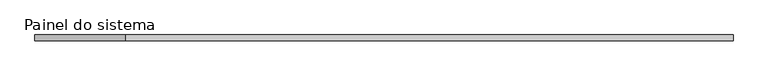
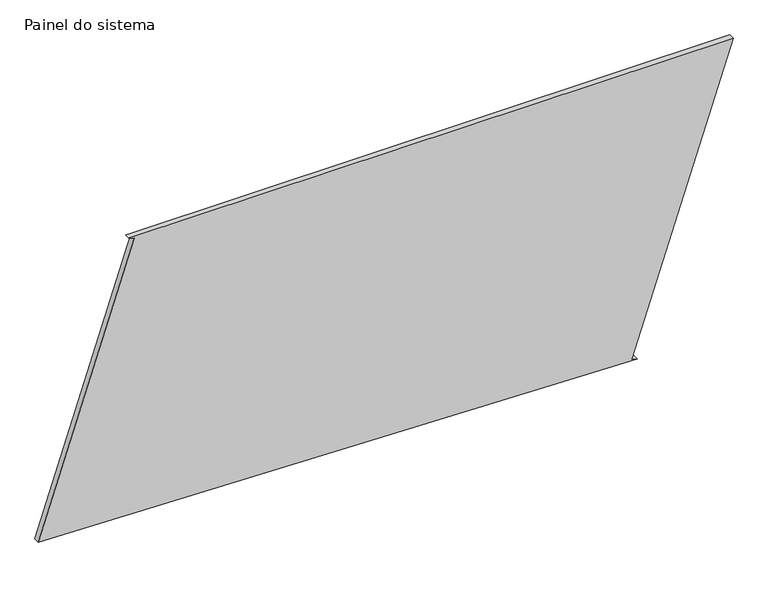
"""IFC4 building model written with IfcOpenShell, lengths in millimetres: plate geometry, Painel do sistema : Envidraçado."""

from ifc_helpers import new_model, si_unit, frame, origin, place, context, project, spatial, polyline, outline, extrude, source, transform, mapped, element, save


def painel_do_sistema_824a56c0(model_context):
    return source(origin(), model_context, "Body", "SweptSolid", [
        extrude(outline(polyline([(0.0, 1117.9483187), (7.8961296, 1094.2280502), (1358.6587643, 1543.8771291), (1358.6587643, -1141.1988644), (1350.7626347, -1117.4785959), (69.8455081, -1543.8771291), (0.0, 1117.9483187)])), frame((0.0, 24.5, 0.0), z_axis=(0.0, 1.0, 0.0), x_axis=(0.0, 0.0, 1.0)), (0.0, 0.0, 1.0), 25.0),
    ])


if __name__ == "__main__":
    model = new_model("IFC4")
    model_context = context("Model", 3, world=origin())
    ifc_project = project(units=[si_unit("LENGTHUNIT", "METRE", prefix="MILLI")], contexts=[model_context])
    site = spatial("IfcSite", under=ifc_project)
    building = spatial("IfcBuilding", under=site)
    placement = place(None, origin())
    painel_do_sistema_shape = painel_do_sistema_824a56c0(model_context)
    element("IfcPlate", 1, ObjectType="Painel do sistema : Envidraçado", at=placement, inside=building, context=model_context, shape_type="MappedRepresentation", body=[
        mapped(painel_do_sistema_shape, transform((0.0, 0.0, 0.0), x_axis=(1.0, 0.0, 0.0), y_axis=(0.0, 1.0, 0.0), z_axis=(0.0, 0.0, 1.0))),
    ])
    save(model, "model.ifc")

# Revit data of these elements
# Type "Painel do sistema : Envidraçado"
#   Construction Type Id = "GSP4R"
#   Analytic Construction = "Vidraça única Pilkington 1/8 pol"
#   Visual Light Transmittance = 0.9
#   Solar Heat Gain Coefficient = 0.86
#   Heat Transfer Coefficient (U) = 6.7069 W/(m²·K)
# Element 1 (IfcPlate, "Painel do sistema : Envidraçado")
#   Materials on its faces: "Vidro"
# Materials
#   "Vidro": class "Vidro", colour RGB 0 128 192, transparency 0.9, Description = "Vidro de sílica", Cost = 0
